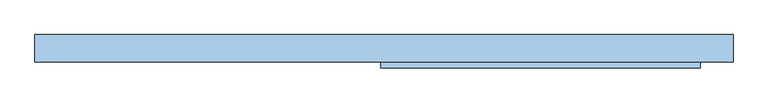
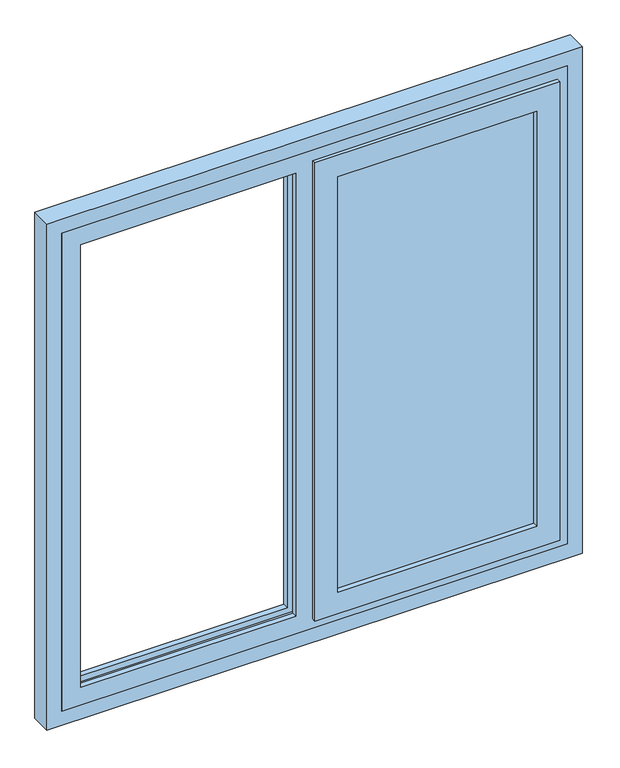
"""IFC4 building model written with IfcOpenShell, lengths in millimetres: window geometry, Окно 2-Откидное - Левое глухое - Один переплет с многокамерным стеклопакетом - 30674-99 : ОП Г1760-1770 (4M1-10-4M1-10-4M1) ГОСТ 30674-99."""

import ifcopenshell
import ifcopenshell.guid

model = None  # the IFC model being written
_history = None  # IfcOwnerHistory: only IFC2X3 demands one
_inside = {}  # id of a spatial element -> (the spatial element, [elements in it])
_under = {}  # id of a project, library or spatial element -> (it, [spatial elements below it])
_declared = {}  # id of a project -> (the project, [libraries it declares])
_typed = {}  # id of a type object -> (the type object, [elements of that type])
_made_of = {}  # id of a material, layer set ... -> (it, [elements and type objects made of it])


def new_model(schema):
    """Start an empty IFC model of exactly this schema.

    Asked for "IFC4X3", IfcOpenShell would pick the latest addendum, in which some entities
    have other attributes; the version numbers below select the first issue.
    IFC2X3 requires an IfcOwnerHistory on every rooted entity: one is made here for all.
    """
    global model, _history
    if schema == "IFC4X3":
        model = ifcopenshell.file(schema_version=(4, 3, 0, 0))
    else:
        model = ifcopenshell.file(schema=schema)
    _inside.clear()
    _under.clear()
    _declared.clear()
    _typed.clear()
    _made_of.clear()
    _history = None
    if model.schema == "IFC2X3":
        org = make("IfcOrganization", Name="unknown")
        user = make(
            "IfcPersonAndOrganization",
            ThePerson=make("IfcPerson", FamilyName="unknown"),
            TheOrganization=org,
        )
        app = make(
            "IfcApplication",
            ApplicationDeveloper=org,
            Version="unknown",
            ApplicationFullName="unknown",
            ApplicationIdentifier="unknown",
        )
        _history = make(
            "IfcOwnerHistory",
            OwningUser=user,
            OwningApplication=app,
            ChangeAction="ADDED",
            CreationDate=0,
        )
    return model


def make(cls, **values):
    """One entity of the class cls with the attributes given. An attribute that is None is left unset."""
    return model.create_entity(
        cls, **{name: value for name, value in values.items() if value is not None}
    )


def rooted(cls, **values):
    """An entity with a GlobalId (a new one), such as an element, a storey or a relation."""
    return make(cls, GlobalId=ifcopenshell.guid.new(), OwnerHistory=_history, **values)


def si_unit(unit_type, name, prefix=None):
    """IfcSIUnit, for example si_unit("LENGTHUNIT", "METRE", prefix="MILLI")."""
    return make("IfcSIUnit", UnitType=unit_type, Prefix=prefix, Name=name)


def assignment(units):
    """IfcUnitAssignment: the units of a project."""
    return None if units is None else make("IfcUnitAssignment", Units=units)


def point(xyz):
    """IfcCartesianPoint."""
    return None if xyz is None else make("IfcCartesianPoint", Coordinates=xyz)


def direction(xyz):
    """IfcDirection."""
    return None if xyz is None else make("IfcDirection", DirectionRatios=xyz)


def frame(location, z_axis=None, x_axis=None):
    """IfcAxis2Placement3D, a coordinate frame: its origin and axes. An axis left out is left unset."""
    return make(
        "IfcAxis2Placement3D",
        Location=point(location),
        Axis=direction(z_axis),
        RefDirection=direction(x_axis),
    )


def origin():
    """The frame at (0, 0, 0) with its axes left unset."""
    return frame((0.0, 0.0, 0.0))


def place(relative_to, where):
    """IfcLocalPlacement: puts the frame where relative to a parent placement (None: the world)."""
    return make(
        "IfcLocalPlacement", PlacementRelTo=relative_to, RelativePlacement=where
    )


def context(
    kind, dimensions, precision=None, world=None, true_north=None, identifier=None
):
    """IfcGeometricRepresentationContext, for example the 3D "Model" context."""
    return make(
        "IfcGeometricRepresentationContext",
        ContextIdentifier=identifier,
        ContextType=kind,
        CoordinateSpaceDimension=dimensions,
        Precision=precision,
        WorldCoordinateSystem=world,
        TrueNorth=true_north,
    )


def project(units=None, contexts=None):
    """IfcProject with its units and contexts."""
    return rooted(
        "IfcProject",
        Name="project",
        RepresentationContexts=contexts,
        UnitsInContext=assignment(units),
    )


def spatial(cls, under=None, at=None, **own):
    """A site, building, storey or space (cls), placed at a placement, below another one or the project."""
    s = rooted(cls, ObjectPlacement=at, **own)
    if under is not None:
        _under.setdefault(under.id(), (under, []))[1].append(s)
    return s


def polyline(points):
    """IfcPolyline through the points."""
    return make("IfcPolyline", Points=[point(p) for p in points])


def outline(outer, holes=None, kind="AREA"):
    """IfcArbitraryClosedProfileDef: a profile drawn as a closed curve; with holes, ...WithVoids."""
    if holes is None:
        return make("IfcArbitraryClosedProfileDef", ProfileType=kind, OuterCurve=outer)
    return make(
        "IfcArbitraryProfileDefWithVoids",
        ProfileType=kind,
        OuterCurve=outer,
        InnerCurves=holes,
    )


def extrude(swept, where, along, depth):
    """IfcExtrudedAreaSolid: the profile swept, set in the frame where, extruded along a direction by depth."""
    return make(
        "IfcExtrudedAreaSolid",
        SweptArea=swept,
        Position=where,
        ExtrudedDirection=direction(along),
        Depth=depth,
    )


def faces_of(points, faces, orient=None, outer=None):
    """IfcFace entities. A face is a list of loops; a loop is a list of indices into points, from 0.

    orient and outer hold one flag for each loop. By default every Orientation is true, the
    first loop of a face is its IfcFaceOuterBound and the others are IfcFaceBound.
    """
    made = []
    for i, loops in enumerate(faces):
        bounds = []
        for j, loop in enumerate(loops):
            is_outer = j == 0 if outer is None else outer[i][j]
            bounds.append(
                make(
                    "IfcFaceOuterBound" if is_outer else "IfcFaceBound",
                    Bound=make("IfcPolyLoop", Polygon=[points[k] for k in loop]),
                    Orientation=True if orient is None else orient[i][j],
                )
            )
        made.append(make("IfcFace", Bounds=bounds))
    return made


def faceted_brep(points, faces, orient=None, outer=None, voids=None):
    """IfcFacetedBrep: a solid bounded by flat faces; with voids (closed shells), ...WithVoids."""
    shared = [point(p) for p in points]
    hull = make("IfcClosedShell", CfsFaces=faces_of(shared, faces, orient, outer))
    if voids is None:
        return make("IfcFacetedBrep", Outer=hull)
    return make(
        "IfcFacetedBrepWithVoids",
        Outer=hull,
        Voids=[
            make(cls, CfsFaces=faces_of(shared, fs, o, b)) for cls, fs, o, b in voids
        ],
    )


def shape(context_of_items, identifier, shape_type, items):
    """IfcShapeRepresentation: the items that make up one representation, for example the "Body"."""
    return make(
        "IfcShapeRepresentation",
        ContextOfItems=context_of_items,
        RepresentationIdentifier=identifier,
        RepresentationType=shape_type,
        Items=items,
    )


def source(mapping_origin, context_of_items, identifier, shape_type, items):
    """IfcRepresentationMap: a shape defined once, which mapped items show again and again."""
    return make(
        "IfcRepresentationMap",
        MappingOrigin=mapping_origin,
        MappedRepresentation=shape(context_of_items, identifier, shape_type, items),
    )


def transform(
    local_origin,
    x_axis=None,
    y_axis=None,
    z_axis=None,
    scale=None,
    scale2=None,
    scale3=None,
    uniform=True,
):
    """IfcCartesianTransformationOperator3D, or its non-uniform kind. x_axis, y_axis, z_axis: its Axis1, 2, 3."""
    if uniform:
        return make(
            "IfcCartesianTransformationOperator3D",
            Axis1=direction(x_axis),
            Axis2=direction(y_axis),
            LocalOrigin=point(local_origin),
            Scale=scale,
            Axis3=direction(z_axis),
        )
    return make(
        "IfcCartesianTransformationOperator3DnonUniform",
        Axis1=direction(x_axis),
        Axis2=direction(y_axis),
        LocalOrigin=point(local_origin),
        Scale=scale,
        Axis3=direction(z_axis),
        Scale2=scale2,
        Scale3=scale3,
    )


def mapped(mapping_source, mapping_target):
    """IfcMappedItem: shows the shape of a source again, moved by a transform."""
    return make(
        "IfcMappedItem", MappingSource=mapping_source, MappingTarget=mapping_target
    )


def made_of(thing, what):
    """Note that an element or type object is made of a material, layer set ...; save() writes the relation."""
    if what is not None:
        _made_of.setdefault(what.id(), (what, []))[1].append(thing)
    return thing


def element(
    cls,
    number,
    at=None,
    inside=None,
    cuts=None,
    type_object=None,
    material=None,
    context=None,
    identifier="Body",
    shape_type=None,
    held_by="IfcProductDefinitionShape",
    body=None,
    shapes=None,
    **own,
):
    """One element of the class cls, such as IfcWall. Its Tag is "e" and its number.

    at: its placement. inside: the storey or other place that contains it. cuts: it is an
    opening in that element (IfcRelVoidsElement). A single representation is given by context,
    identifier, shape_type and body (its items); several are given by shapes. held_by: the class
    of the entity that holds the representations. save() writes the other relations.
    """
    e = rooted(cls, Tag="e%d" % number, ObjectPlacement=at, **own)
    if body is not None:
        shapes = [shape(context, identifier, shape_type, body)]
    if shapes is not None:
        e.Representation = make(held_by, Representations=shapes)
    if inside is not None:
        _inside.setdefault(inside.id(), (inside, []))[1].append(e)
    if cuts is not None:
        rooted(
            "IfcRelVoidsElement", RelatingBuildingElement=cuts, RelatedOpeningElement=e
        )
    if type_object is not None:
        _typed.setdefault(type_object.id(), (type_object, []))[1].append(e)
    return made_of(e, material)


def aggregate(whole, parts):
    """IfcRelAggregates: a whole, such as a stair, and the parts it consists of."""
    return rooted("IfcRelAggregates", RelatingObject=whole, RelatedObjects=parts)


def save(model, path):
    """Write the relations noted so far, then the file.

    IfcRelAggregates (storeys below a building ...), IfcRelContainedInSpatialStructure (elements
    in a storey), IfcRelDefinesByType, IfcRelAssociatesMaterial and IfcRelDeclares: one each for
    every whole, place, type object, material and project.
    """
    for whole, parts in _under.values():
        aggregate(whole, parts)
    for where, things in _inside.values():
        rooted(
            "IfcRelContainedInSpatialStructure",
            RelatedElements=things,
            RelatingStructure=where,
        )
    for kind, things in _typed.values():
        rooted("IfcRelDefinesByType", RelatedObjects=things, RelatingType=kind)
    for what, things in _made_of.values():
        rooted("IfcRelAssociatesMaterial", RelatedObjects=things, RelatingMaterial=what)
    for by, libraries in _declared.values():
        rooted("IfcRelDeclares", RelatingContext=by, RelatedDefinitions=libraries)
    model.write(path)


def window_c31c645a(model_context):
    return source(origin(), model_context, "Body", "SolidModel", [
        extrude(outline(polyline([(942.0, 758.0), (2458.0, 758.0), (2458.0, 49.0), (942.0, 49.0), (942.0, 758.0)]), holes=[polyline([(2443.0, 743.0), (957.0, 743.0), (957.0, 64.0), (2443.0, 64.0), (2443.0, 743.0)])]), frame((0.0, 25.0, 0.0), z_axis=(0.0, 1.0, 0.0), x_axis=(0.0, 0.0, 1.0)), (0.0, 0.0, 1.0), 10.0),
        extrude(outline(polyline([(942.0, 758.0), (2458.0, 758.0), (2458.0, 49.0), (942.0, 49.0), (942.0, 758.0)]), holes=[polyline([(2443.0, 743.0), (957.0, 743.0), (957.0, 64.0), (2443.0, 64.0), (2443.0, 743.0)])]), frame((0.0, 11.0, 0.0), z_axis=(0.0, 1.0, 0.0), x_axis=(0.0, 0.0, 1.0)), (0.0, 0.0, 1.0), 10.0),
        extrude(outline(polyline([(49.0, 25.0), (758.0, 25.0), (758.0, 21.0), (49.0, 21.0), (49.0, 25.0)])), frame((0.0, 0.0, 942.0), z_axis=(0.0, 0.0, 1.0), x_axis=(1.0, 0.0, 0.0)), (0.0, 0.0, 1.0), 1516.0),
        extrude(outline(polyline([(49.0, 39.0), (758.0, 39.0), (758.0, 35.0), (49.0, 35.0), (49.0, 39.0)])), frame((0.0, 0.0, 942.0), z_axis=(0.0, 0.0, 1.0), x_axis=(1.0, 0.0, 0.0)), (0.0, 0.0, 1.0), 1516.0),
        extrude(outline(polyline([(49.0, 11.0), (758.0, 11.0), (758.0, 7.0), (49.0, 7.0), (49.0, 11.0)])), frame((0.0, 0.0, 942.0), z_axis=(0.0, 0.0, 1.0), x_axis=(1.0, 0.0, 0.0)), (0.0, 0.0, 1.0), 1516.0),
        faceted_brep([(-850.0, 5.0, 2550.0), (-850.0, 75.0, 2550.0), (-850.0, 75.0, 850.0), (-850.0, 5.0, 850.0), (850.0, 75.0, 850.0), (850.0, 75.0, 2550.0), (-787.0, 75.0, 2487.0), (-787.0, 75.0, 913.0), (-63.0, 75.0, 913.0), (-63.0, 75.0, 2487.0), (19.0, 75.0, 2487.0), (19.0, 75.0, 913.0), (787.0, 75.0, 913.0), (787.0, 75.0, 2487.0), (850.0, 5.0, 850.0), (850.0, 5.0, 2550.0), (-787.0, 5.0, 913.0), (-787.0, 5.0, 2487.0), (-63.0, 5.0, 2487.0), (-63.0, 5.0, 913.0), (0.0, 5.0, 893.0), (0.0, 5.0, 2507.0), (807.0, 5.0, 2507.0), (807.0, 5.0, 893.0), (-787.0, 23.0, 2487.0), (-787.0, 23.0, 913.0), (-63.0, 23.0, 913.0), (-807.0, 23.0, 893.0), (-807.0, 23.0, 2507.0), (-43.0, 23.0, 2507.0), (-43.0, 23.0, 893.0), (-63.0, 23.0, 2487.0), (-807.0, 55.0, 2507.0), (-807.0, 55.0, 893.0), (-43.0, 55.0, 893.0), (-43.0, 55.0, 2507.0), (-787.0, 55.0, 913.0), (-787.0, 55.0, 2487.0), (-63.0, 55.0, 2487.0), (-63.0, 55.0, 913.0), (0.0, 61.0, 893.0), (0.0, 61.0, 2507.0), (807.0, 61.0, 893.0), (807.0, 61.0, 2507.0), (19.0, 61.0, 913.0), (19.0, 61.0, 2487.0), (787.0, 61.0, 2487.0), (787.0, 61.0, 913.0)], [[[0, 1, 2, 3]], [[4, 2, 1, 5], [6, 7, 8, 9], [10, 11, 12, 13]], [[3, 2, 4, 14]], [[15, 0, 3, 14], [16, 17, 18, 19], [20, 21, 22, 23]], [[24, 17, 16, 25]], [[25, 16, 19, 26]], [[27, 28, 29, 30], [24, 25, 26, 31]], [[32, 28, 27, 33]], [[33, 27, 30, 34]], [[32, 33, 34, 35], [36, 37, 38, 39]], [[6, 37, 36, 7]], [[7, 36, 39, 8]], [[15, 14, 4, 5]], [[26, 19, 18, 31]], [[34, 30, 29, 35]], [[8, 39, 38, 9]], [[40, 41, 21, 20]], [[42, 43, 41, 40], [44, 45, 46, 47]], [[20, 23, 42, 40]], [[11, 10, 45, 44]], [[47, 12, 11, 44]], [[46, 13, 12, 47]], [[43, 42, 23, 22]], [[5, 1, 0, 15]], [[17, 24, 31, 18]], [[28, 32, 35, 29]], [[37, 6, 9, 38]], [[13, 46, 45, 10]], [[41, 43, 22, 21]]]),
        faceted_brep([(69.0, 59.0, 2438.0), (69.0, 39.0, 2438.0), (69.0, 39.0, 962.0), (69.0, 59.0, 962.0), (49.0, 39.0, 942.0), (758.0, 39.0, 942.0), (758.0, 39.0, 2458.0), (49.0, 39.0, 2458.0), (738.0, 39.0, 2438.0), (738.0, 39.0, 962.0), (738.0, 59.0, 962.0), (12.0, 59.0, 2495.0), (795.0, 59.0, 2495.0), (795.0, 59.0, 905.0), (12.0, 59.0, 905.0), (738.0, 59.0, 2438.0), (12.0, 3.0, 2495.0), (12.0, 3.0, 905.0), (795.0, 3.0, 905.0), (-8.0, 3.0, 2515.0), (815.0, 3.0, 2515.0), (815.0, 3.0, 885.0), (-8.0, 3.0, 885.0), (795.0, 3.0, 2495.0), (-8.0, -11.0, 2515.0), (-8.0, -11.0, 885.0), (815.0, -11.0, 885.0), (815.0, -11.0, 2515.0), (69.0, -11.0, 2438.0), (738.0, -11.0, 2438.0), (738.0, -11.0, 962.0), (69.0, -11.0, 962.0), (69.0, 7.0, 2438.0), (69.0, 7.0, 962.0), (738.0, 7.0, 962.0), (49.0, 7.0, 2458.0), (758.0, 7.0, 2458.0), (758.0, 7.0, 942.0), (49.0, 7.0, 942.0), (738.0, 7.0, 2438.0)], [[[0, 1, 2, 3]], [[4, 5, 6, 7], [1, 8, 9, 2]], [[3, 2, 9, 10]], [[11, 12, 13, 14], [3, 10, 15, 0]], [[16, 11, 14, 17]], [[17, 14, 13, 18]], [[19, 20, 21, 22], [17, 18, 23, 16]], [[24, 19, 22, 25]], [[25, 22, 21, 26]], [[25, 26, 27, 24], [28, 29, 30, 31]], [[32, 28, 31, 33]], [[33, 31, 30, 34]], [[35, 36, 37, 38], [33, 34, 39, 32]], [[7, 35, 38, 4]], [[4, 38, 37, 5]], [[10, 9, 8, 15]], [[18, 13, 12, 23]], [[26, 21, 20, 27]], [[34, 30, 29, 39]], [[5, 37, 36, 6]], [[15, 8, 1, 0]], [[23, 12, 11, 16]], [[27, 20, 19, 24]], [[39, 29, 28, 32]], [[6, 36, 35, 7]]]),
        extrude(outline(polyline([(800.0, -900.0), (800.0, 900.0), (2600.0, 900.0), (2600.0, -900.0), (800.0, -900.0)]), holes=[polyline([(2550.0, -850.0), (2550.0, 850.0), (850.0, 850.0), (850.0, -850.0), (2550.0, -850.0)])]), frame((0.0, 5.0, 0.0), z_axis=(0.0, 1.0, 0.0), x_axis=(0.0, 0.0, 1.0)), (0.0, 0.0, 1.0), 70.0),
    ])


if __name__ == "__main__":
    model = new_model("IFC4")
    model_context = context("Model", 3, world=origin())
    ifc_project = project(units=[si_unit("LENGTHUNIT", "METRE", prefix="MILLI")], contexts=[model_context])
    site = spatial("IfcSite", under=ifc_project)
    building = spatial("IfcBuilding", under=site)
    placement = place(None, origin())
    window_shape = window_c31c645a(model_context)
    element("IfcWindow", 1, ObjectType="Окно 2-Откидное - Левое глухое - Один переплет с многокамерным стеклопакетом - 30674-99 : ОП Г1760-1770 (4M1-10-4M1-10-4M1) ГОСТ 30674-99", at=placement, inside=building, context=model_context, shape_type="MappedRepresentation", body=[
        mapped(window_shape, transform((0.0, 0.0, 0.0), x_axis=(1.0, 0.0, 0.0), y_axis=(0.0, 1.0, 0.0), z_axis=(0.0, 0.0, 1.0))),
    ])
    save(model, "model.ifc")

# Revit data of these elements
# Type "Окно 2-Откидное - Левое глухое - Один переплет с многокамерным стеклопакетом - 30674-99 : ОП Г1760-1770 (4M1-10-4M1-10-4M1) ГОСТ 30674-99"
#   Type Mark = "108"
#   Description = "ОП Г1  1200-1400 (4M1-10-4M1-10-4M1) ГОСТ 30674-99"
#   Вставка окна [instance default] = 0 mm
#   Visual Light Transmittance = 0.9
#   Solar Heat Gain Coefficient = 0.78
#   Ширина переплета 1 = 77 mm
#   Rough Width = 1800 mm
#   Rough Height = 1800 mm
#   Height = 1700 mm
#   Толщина_Тепл_Изоляции = 50 mm
#   Heat Transfer Coefficient (U) = 3.6886 W/(m²·K)
#   G = 32 mm
#   Ширина каркаса = 63 mm
#   Высота подоконника по умолчанию = 800 mm
#   Width = 1700 mm
#   Трехкамерный стеклопакет = yes
#   Двухкамерный стеклопакет = no
#   Переплет = Деревянный переплет
#   Тепловая изоляция = Тепловая изоляция
#   Оконное стекло = Стекло
#   Кадр = Деревянный каркас
#   Construction Type Id = ""
#   Wall Closure = (empty or 0)
#   Analytic Construction = (empty or 0)
# Element 1 (IfcWindow, "Окно 2-Откидное - Левое глухое - Один переплет с многокамерным стеклопакетом - 30674-99 : ОП Г1760-1770 (4M1-10-4M1-10-4M1) ГОСТ 30674-99")
#   Materials on its faces: "Деревянный каркас", "Деревянный переплет", "Алюминий", "Стекло", "Тепловая изоляция"
# Materials
#   "Деревянный переплет": class "Древесина", colour RGB 224 176 126, transparency 0, Cost = 0
#   "Тепловая изоляция": class "Пластмасса", colour RGB 185 154 119, transparency 0, Cost = 0
#   "Стекло": class "Стекло", colour RGB 0 0 255, transparency 0.75
#   "Деревянный каркас": class "Древесина", colour RGB 224 176 126, transparency 0, Cost = 0
#   "Алюминий": class "Металл", colour RGB 247 247 247, transparency 0
